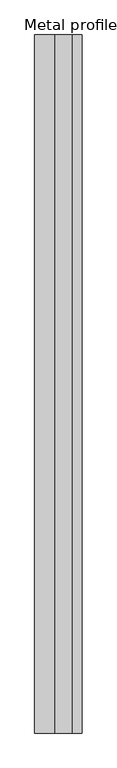
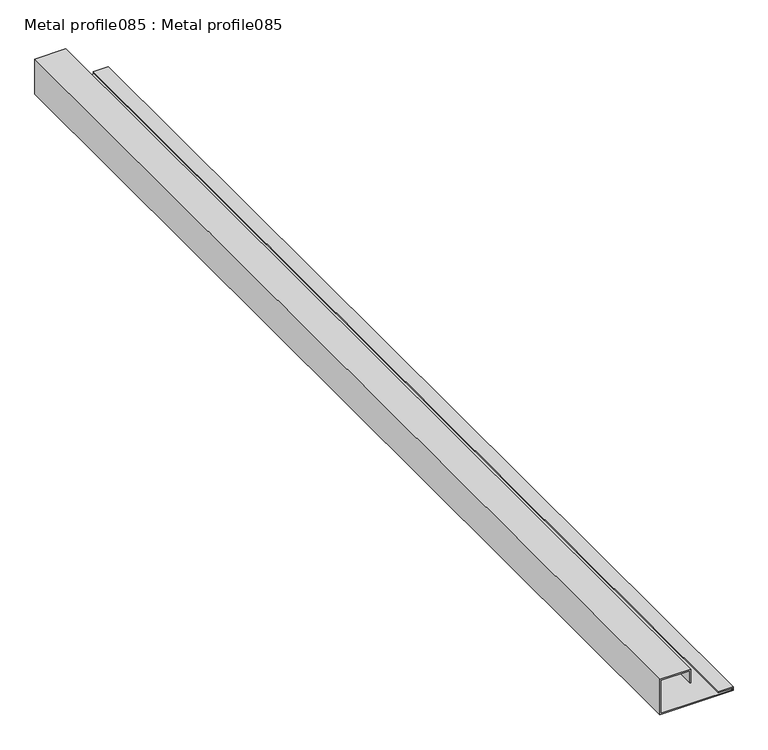
"""IFC4 building model written with IfcOpenShell, lengths in millimetres: proxy geometry, Metal profile085 : Metal profile085."""

import ifcopenshell
import ifcopenshell.guid

model = None  # the IFC model being written
_history = None  # IfcOwnerHistory: only IFC2X3 demands one
_inside = {}  # id of a spatial element -> (the spatial element, [elements in it])
_under = {}  # id of a project, library or spatial element -> (it, [spatial elements below it])
_declared = {}  # id of a project -> (the project, [libraries it declares])
_typed = {}  # id of a type object -> (the type object, [elements of that type])
_made_of = {}  # id of a material, layer set ... -> (it, [elements and type objects made of it])


def new_model(schema):
    """Start an empty IFC model of exactly this schema.

    Asked for "IFC4X3", IfcOpenShell would pick the latest addendum, in which some entities
    have other attributes; the version numbers below select the first issue.
    IFC2X3 requires an IfcOwnerHistory on every rooted entity: one is made here for all.
    """
    global model, _history
    if schema == "IFC4X3":
        model = ifcopenshell.file(schema_version=(4, 3, 0, 0))
    else:
        model = ifcopenshell.file(schema=schema)
    _inside.clear()
    _under.clear()
    _declared.clear()
    _typed.clear()
    _made_of.clear()
    _history = None
    if model.schema == "IFC2X3":
        org = make("IfcOrganization", Name="unknown")
        user = make(
            "IfcPersonAndOrganization",
            ThePerson=make("IfcPerson", FamilyName="unknown"),
            TheOrganization=org,
        )
        app = make(
            "IfcApplication",
            ApplicationDeveloper=org,
            Version="unknown",
            ApplicationFullName="unknown",
            ApplicationIdentifier="unknown",
        )
        _history = make(
            "IfcOwnerHistory",
            OwningUser=user,
            OwningApplication=app,
            ChangeAction="ADDED",
            CreationDate=0,
        )
    return model


def make(cls, **values):
    """One entity of the class cls with the attributes given. An attribute that is None is left unset."""
    return model.create_entity(
        cls, **{name: value for name, value in values.items() if value is not None}
    )


def rooted(cls, **values):
    """An entity with a GlobalId (a new one), such as an element, a storey or a relation."""
    return make(cls, GlobalId=ifcopenshell.guid.new(), OwnerHistory=_history, **values)


def si_unit(unit_type, name, prefix=None):
    """IfcSIUnit, for example si_unit("LENGTHUNIT", "METRE", prefix="MILLI")."""
    return make("IfcSIUnit", UnitType=unit_type, Prefix=prefix, Name=name)


def assignment(units):
    """IfcUnitAssignment: the units of a project."""
    return None if units is None else make("IfcUnitAssignment", Units=units)


def point(xyz):
    """IfcCartesianPoint."""
    return None if xyz is None else make("IfcCartesianPoint", Coordinates=xyz)


def direction(xyz):
    """IfcDirection."""
    return None if xyz is None else make("IfcDirection", DirectionRatios=xyz)


def frame(location, z_axis=None, x_axis=None):
    """IfcAxis2Placement3D, a coordinate frame: its origin and axes. An axis left out is left unset."""
    return make(
        "IfcAxis2Placement3D",
        Location=point(location),
        Axis=direction(z_axis),
        RefDirection=direction(x_axis),
    )


def origin():
    """The frame at (0, 0, 0) with its axes left unset."""
    return frame((0.0, 0.0, 0.0))


def place(relative_to, where):
    """IfcLocalPlacement: puts the frame where relative to a parent placement (None: the world)."""
    return make(
        "IfcLocalPlacement", PlacementRelTo=relative_to, RelativePlacement=where
    )


def context(
    kind, dimensions, precision=None, world=None, true_north=None, identifier=None
):
    """IfcGeometricRepresentationContext, for example the 3D "Model" context."""
    return make(
        "IfcGeometricRepresentationContext",
        ContextIdentifier=identifier,
        ContextType=kind,
        CoordinateSpaceDimension=dimensions,
        Precision=precision,
        WorldCoordinateSystem=world,
        TrueNorth=true_north,
    )


def project(units=None, contexts=None):
    """IfcProject with its units and contexts."""
    return rooted(
        "IfcProject",
        Name="project",
        RepresentationContexts=contexts,
        UnitsInContext=assignment(units),
    )


def spatial(cls, under=None, at=None, **own):
    """A site, building, storey or space (cls), placed at a placement, below another one or the project."""
    s = rooted(cls, ObjectPlacement=at, **own)
    if under is not None:
        _under.setdefault(under.id(), (under, []))[1].append(s)
    return s


def polyline(points):
    """IfcPolyline through the points."""
    return make("IfcPolyline", Points=[point(p) for p in points])


def outline(outer, holes=None, kind="AREA"):
    """IfcArbitraryClosedProfileDef: a profile drawn as a closed curve; with holes, ...WithVoids."""
    if holes is None:
        return make("IfcArbitraryClosedProfileDef", ProfileType=kind, OuterCurve=outer)
    return make(
        "IfcArbitraryProfileDefWithVoids",
        ProfileType=kind,
        OuterCurve=outer,
        InnerCurves=holes,
    )


def extrude(swept, where, along, depth):
    """IfcExtrudedAreaSolid: the profile swept, set in the frame where, extruded along a direction by depth."""
    return make(
        "IfcExtrudedAreaSolid",
        SweptArea=swept,
        Position=where,
        ExtrudedDirection=direction(along),
        Depth=depth,
    )


def shape(context_of_items, identifier, shape_type, items):
    """IfcShapeRepresentation: the items that make up one representation, for example the "Body"."""
    return make(
        "IfcShapeRepresentation",
        ContextOfItems=context_of_items,
        RepresentationIdentifier=identifier,
        RepresentationType=shape_type,
        Items=items,
    )


def source(mapping_origin, context_of_items, identifier, shape_type, items):
    """IfcRepresentationMap: a shape defined once, which mapped items show again and again."""
    return make(
        "IfcRepresentationMap",
        MappingOrigin=mapping_origin,
        MappedRepresentation=shape(context_of_items, identifier, shape_type, items),
    )


def transform(
    local_origin,
    x_axis=None,
    y_axis=None,
    z_axis=None,
    scale=None,
    scale2=None,
    scale3=None,
    uniform=True,
):
    """IfcCartesianTransformationOperator3D, or its non-uniform kind. x_axis, y_axis, z_axis: its Axis1, 2, 3."""
    if uniform:
        return make(
            "IfcCartesianTransformationOperator3D",
            Axis1=direction(x_axis),
            Axis2=direction(y_axis),
            LocalOrigin=point(local_origin),
            Scale=scale,
            Axis3=direction(z_axis),
        )
    return make(
        "IfcCartesianTransformationOperator3DnonUniform",
        Axis1=direction(x_axis),
        Axis2=direction(y_axis),
        LocalOrigin=point(local_origin),
        Scale=scale,
        Axis3=direction(z_axis),
        Scale2=scale2,
        Scale3=scale3,
    )


def mapped(mapping_source, mapping_target):
    """IfcMappedItem: shows the shape of a source again, moved by a transform."""
    return make(
        "IfcMappedItem", MappingSource=mapping_source, MappingTarget=mapping_target
    )


def made_of(thing, what):
    """Note that an element or type object is made of a material, layer set ...; save() writes the relation."""
    if what is not None:
        _made_of.setdefault(what.id(), (what, []))[1].append(thing)
    return thing


def element(
    cls,
    number,
    at=None,
    inside=None,
    cuts=None,
    type_object=None,
    material=None,
    context=None,
    identifier="Body",
    shape_type=None,
    held_by="IfcProductDefinitionShape",
    body=None,
    shapes=None,
    **own,
):
    """One element of the class cls, such as IfcWall. Its Tag is "e" and its number.

    at: its placement. inside: the storey or other place that contains it. cuts: it is an
    opening in that element (IfcRelVoidsElement). A single representation is given by context,
    identifier, shape_type and body (its items); several are given by shapes. held_by: the class
    of the entity that holds the representations. save() writes the other relations.
    """
    e = rooted(cls, Tag="e%d" % number, ObjectPlacement=at, **own)
    if body is not None:
        shapes = [shape(context, identifier, shape_type, body)]
    if shapes is not None:
        e.Representation = make(held_by, Representations=shapes)
    if inside is not None:
        _inside.setdefault(inside.id(), (inside, []))[1].append(e)
    if cuts is not None:
        rooted(
            "IfcRelVoidsElement", RelatingBuildingElement=cuts, RelatedOpeningElement=e
        )
    if type_object is not None:
        _typed.setdefault(type_object.id(), (type_object, []))[1].append(e)
    return made_of(e, material)


def aggregate(whole, parts):
    """IfcRelAggregates: a whole, such as a stair, and the parts it consists of."""
    return rooted("IfcRelAggregates", RelatingObject=whole, RelatedObjects=parts)


def save(model, path):
    """Write the relations noted so far, then the file.

    IfcRelAggregates (storeys below a building ...), IfcRelContainedInSpatialStructure (elements
    in a storey), IfcRelDefinesByType, IfcRelAssociatesMaterial and IfcRelDeclares: one each for
    every whole, place, type object, material and project.
    """
    for whole, parts in _under.values():
        aggregate(whole, parts)
    for where, things in _inside.values():
        rooted(
            "IfcRelContainedInSpatialStructure",
            RelatedElements=things,
            RelatingStructure=where,
        )
    for kind, things in _typed.values():
        rooted("IfcRelDefinesByType", RelatedObjects=things, RelatingType=kind)
    for what, things in _made_of.values():
        rooted("IfcRelAssociatesMaterial", RelatedObjects=things, RelatingMaterial=what)
    for by, libraries in _declared.values():
        rooted("IfcRelDeclares", RelatingContext=by, RelatedDefinitions=libraries)
    model.write(path)


def metal_profile085_metal_profile085_73fac49b(model_context):
    return source(origin(), model_context, "Body", "SweptSolid", [
        extrude(outline(polyline([(42529.5797448, -2355.870033), (42529.5797448, -2330.1068494), (42526.7125573, -2330.1068494), (42526.7125573, -2461.7059705), (42591.4859948, -2461.7059705), (42591.4859948, -2408.3607556), (42567.3922448, -2408.3607556), (42567.3922448, -2406.3607556), (42593.4859948, -2406.3607556), (42593.4859948, -2463.7059705), (42524.7125573, -2463.7059705), (42524.7125573, -2328.1068494), (42531.5797448, -2328.1068494), (42531.5797448, -2355.870033), (42529.5797448, -2355.870033)])), frame((0.0, -1052.8906574, 0.0), z_axis=(0.0, 1.0, 0.0), x_axis=(0.0, 0.0, 1.0)), (0.0, 0.0, 1.0), 2000.0),
    ])


if __name__ == "__main__":
    model = new_model("IFC4")
    model_context = context("Model", 3, world=origin())
    ifc_project = project(units=[si_unit("LENGTHUNIT", "METRE", prefix="MILLI")], contexts=[model_context])
    site = spatial("IfcSite", under=ifc_project)
    building = spatial("IfcBuilding", under=site)
    placement = place(None, origin())
    metal_profile085_metal_profile085_shape = metal_profile085_metal_profile085_73fac49b(model_context)
    element("IfcBuildingElementProxy", 1, Name="Metal profile085 : Metal profile085", ObjectType="Metal profile085 : Metal profile085", at=placement, inside=building, context=model_context, shape_type="MappedRepresentation", body=[
        mapped(metal_profile085_metal_profile085_shape, transform((0.0, 0.0, 0.0), x_axis=(1.0, 0.0, 0.0), y_axis=(0.0, 1.0, 0.0), z_axis=(0.0, 0.0, 1.0))),
    ])
    save(model, "model.ifc")

# Revit data of these elements
# Type "Metal profile085 : Metal profile085"
#   NameOverride = "Metal profile085"
# Element 1 (IfcBuildingElementProxy, "Metal profile085 : Metal profile085")
#   Materials on its faces: "RECEIVER TRIM"
# Materials
#   "RECEIVER TRIM": class "Unassigned", colour RGB 255 250 0, transparency 0
